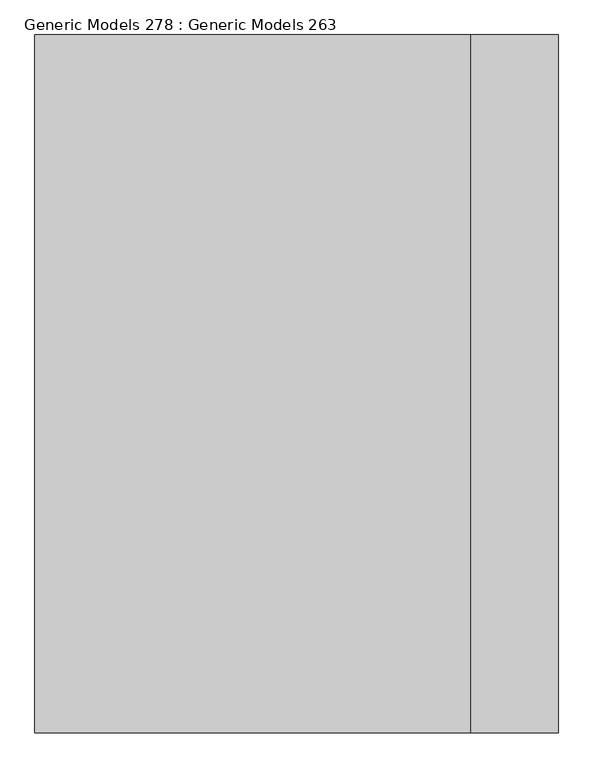
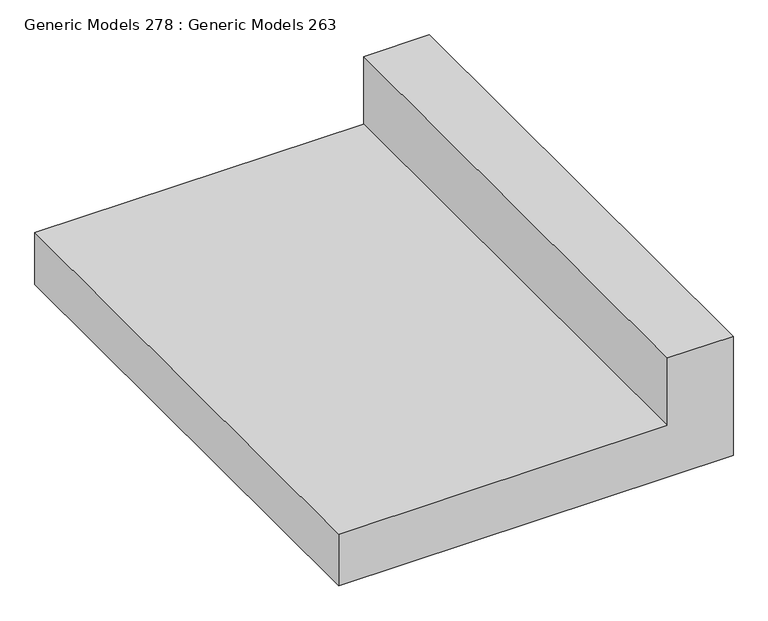
"""IFC4 building model written with IfcOpenShell, lengths in millimetres: proxy geometry, Generic Models 278 : Generic Models 263."""

from ifc_helpers import new_model, si_unit, frame, origin, place, context, project, spatial, polyline, outline, extrude, source, transform, mapped, element, save


def generic_models_278_generic_models_263_5a7632f5(model_context):
    return source(origin(), model_context, "Body", "SweptSolid", [
        extrude(outline(polyline([(-381.0, 60947.5797726), (-381.0, 60185.5797726), (-508.0, 60185.5797726), (-508.0, 61099.9797726), (-215.9, 61099.9797726), (-215.9, 60947.5797726), (-381.0, 60947.5797726)])), frame((0.0, -94.4486541, 0.0), z_axis=(0.0, 1.0, 0.0), x_axis=(0.0, 0.0, 1.0)), (0.0, 0.0, 1.0), 1219.2),
    ])


if __name__ == "__main__":
    model = new_model("IFC4")
    model_context = context("Model", 3, world=origin())
    ifc_project = project(units=[si_unit("LENGTHUNIT", "METRE", prefix="MILLI")], contexts=[model_context])
    site = spatial("IfcSite", under=ifc_project)
    building = spatial("IfcBuilding", under=site)
    placement = place(None, origin())
    generic_models_278_generic_models_263_shape = generic_models_278_generic_models_263_5a7632f5(model_context)
    element("IfcBuildingElementProxy", 1, Name="Generic Models 278 : Generic Models 263", ObjectType="Generic Models 278 : Generic Models 263", at=placement, inside=building, context=model_context, shape_type="MappedRepresentation", body=[
        mapped(generic_models_278_generic_models_263_shape, transform((0.0, 0.0, 0.0), x_axis=(1.0, 0.0, 0.0), y_axis=(0.0, 1.0, 0.0), z_axis=(0.0, 0.0, 1.0))),
    ])
    save(model, "model.ifc")

# Revit data of these elements
# Element 1 (IfcBuildingElementProxy, "Generic Models 278 : Generic Models 263")
#   Materials on its faces: "5\" MIN. COMPACTED BASE AGGREGATE UNDER CURB"
# Materials
#   "5\" MIN. COMPACTED BASE AGGREGATE UNDER CURB": class "Miscellaneous", colour RGB 183 184 198, transparency 0, Cost = 0
